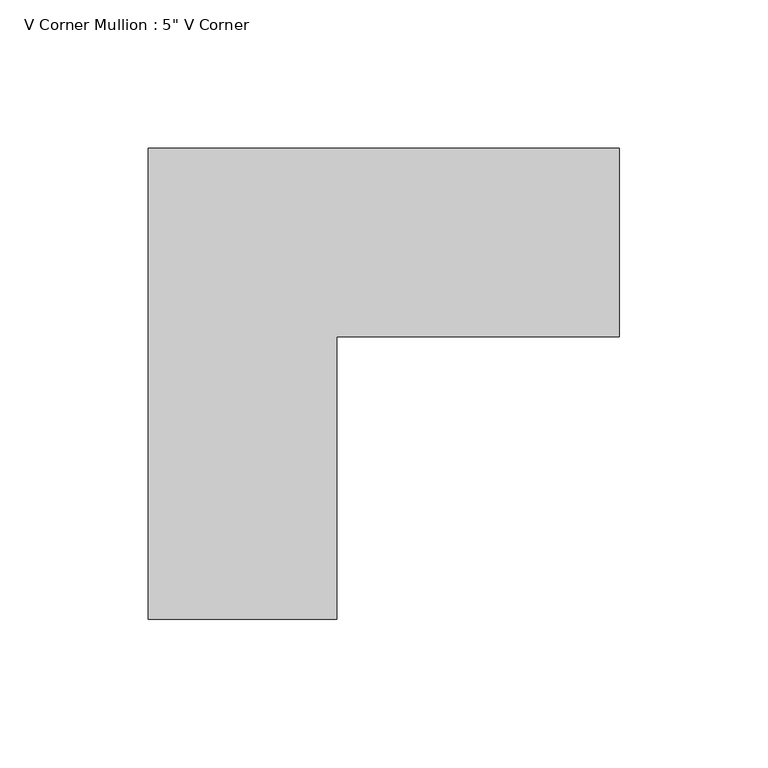
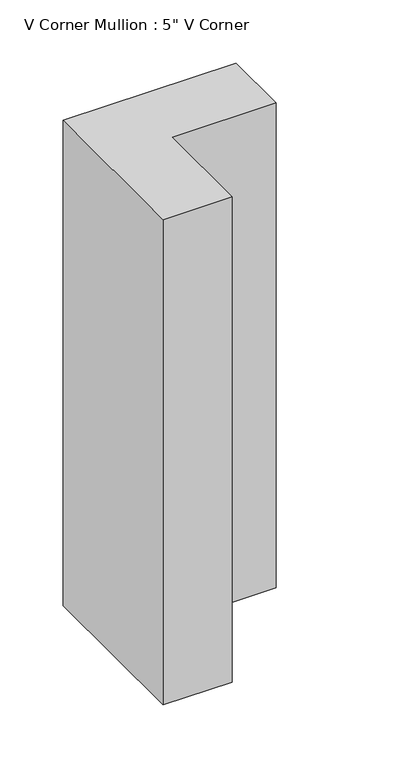
"""IFC4 building model written with IfcOpenShell, lengths in millimetres: member geometry."""

from ifc_helpers import new_model, si_unit, frame, origin, place, context, project, spatial, polyline, outline, extrude, source, transform, mapped, element, save


def member_1dd447f7(model_context):
    return source(origin(), model_context, "Body", "SweptSolid", [
        extrude(outline(polyline([(63.5, 31.75), (-31.75, 31.75), (-31.75, -63.5), (-95.25, -63.5), (-95.25, 95.25), (63.5, 95.25), (63.5, 31.75)])), frame((0.0, 0.0, -469.9), z_axis=(0.0, 0.0, 1.0), x_axis=(1.0, 0.0, 0.0)), (0.0, 0.0, 1.0), 469.9),
    ])


if __name__ == "__main__":
    model = new_model("IFC4")
    model_context = context("Model", 3, world=origin())
    ifc_project = project(units=[si_unit("LENGTHUNIT", "METRE", prefix="MILLI")], contexts=[model_context])
    site = spatial("IfcSite", under=ifc_project)
    building = spatial("IfcBuilding", under=site)
    placement = place(None, origin())
    member_shape = member_1dd447f7(model_context)
    element("IfcMember", 1, ObjectType="V Corner Mullion : 5\" V Corner", at=placement, inside=building, context=model_context, shape_type="MappedRepresentation", body=[
        mapped(member_shape, transform((0.0, 0.0, 0.0), x_axis=(1.0, 0.0, 0.0), y_axis=(0.0, 1.0, 0.0), z_axis=(0.0, 0.0, 1.0))),
    ])
    save(model, "model.ifc")

# Revit data of these elements
# Type "V Corner Mullion : 5\" V Corner"
#   built-in parameter 1007355 = 0.416667 (stored number, unit not read)
#   built-in parameter 1007354 = 0.416667 (stored number, unit not read)
#   built-in parameter 1007304 = 0.208333 (stored number, unit not read)
# Element 1 (IfcMember, "V Corner Mullion : 5\" V Corner")
#   Materials on its faces: "Aluminum"
# Materials
#   "Aluminum": class "Metal", colour RGB 244 245 246, transparency 0, Description = "Aluminum 6061", Cost = 0
